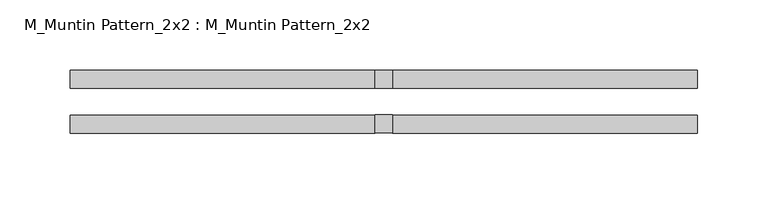
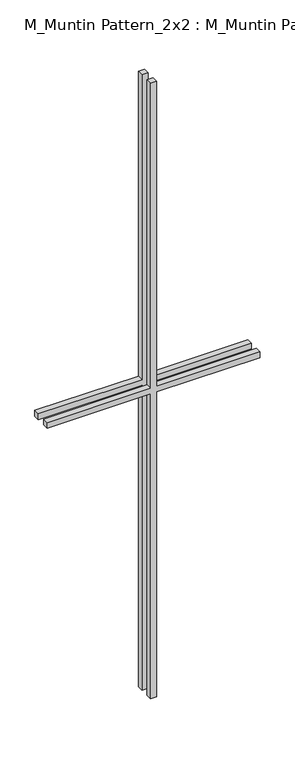
"""IFC4 building model written with IfcOpenShell, lengths in millimetres: proxy geometry, M_Muntin Pattern_2x2 : M_Muntin Pattern_2x2."""

from ifc_helpers import new_model, si_unit, frame, origin, place, context, project, spatial, polyline, outline, extrude, source, transform, mapped, element, save


def m_muntin_pattern_2x2_m_muntin_pattern_2x2_98e5798c(model_context):
    return source(origin(), model_context, "Body", "SweptSolid", [
        extrude(outline(polyline([(686.5, -6.35), (686.5, -223.0), (673.8, -223.0), (673.8, -6.35), (0.0, -6.35), (0.0, 6.35), (673.8, 6.35), (673.8, 223.0), (686.5, 223.0), (686.5, 6.35), (1360.3, 6.35), (1360.3, -6.35), (686.5, -6.35)])), frame((0.0, 9.525, 0.0), z_axis=(0.0, 1.0, 0.0), x_axis=(0.0, 0.0, 1.0)), (0.0, 0.0, 1.0), 12.7),
        extrude(outline(polyline([(686.5, -6.35), (686.5, -223.0), (673.8, -223.0), (673.8, -6.35), (0.0, -6.35), (0.0, 6.35), (673.8, 6.35), (673.8, 223.0), (686.5, 223.0), (686.5, 6.35), (1360.3, 6.35), (1360.3, -6.35), (686.5, -6.35)])), frame((0.0, -22.225, 0.0), z_axis=(0.0, 1.0, 0.0), x_axis=(0.0, 0.0, 1.0)), (0.0, 0.0, 1.0), 12.7),
    ])


if __name__ == "__main__":
    model = new_model("IFC4")
    model_context = context("Model", 3, world=origin())
    ifc_project = project(units=[si_unit("LENGTHUNIT", "METRE", prefix="MILLI")], contexts=[model_context])
    site = spatial("IfcSite", under=ifc_project)
    building = spatial("IfcBuilding", under=site)
    placement = place(None, origin())
    m_muntin_pattern_2x2_m_muntin_pattern_2x2_shape = m_muntin_pattern_2x2_m_muntin_pattern_2x2_98e5798c(model_context)
    element("IfcBuildingElementProxy", 1, Name="M_Muntin Pattern_2x2 : M_Muntin Pattern_2x2", ObjectType="M_Muntin Pattern_2x2 : M_Muntin Pattern_2x2", at=placement, inside=building, context=model_context, shape_type="MappedRepresentation", body=[
        mapped(m_muntin_pattern_2x2_m_muntin_pattern_2x2_shape, transform((0.0, 0.0, 0.0), x_axis=(1.0, 0.0, 0.0), y_axis=(0.0, 1.0, 0.0), z_axis=(0.0, 0.0, 1.0))),
    ])
    save(model, "model.ifc")

# Revit data of these elements
# Type "M_Muntin Pattern_2x2 : M_Muntin Pattern_2x2"
#   Width [instance default] = 1200 mm
#   Thickness = 12.7 mm
#   Height [instance default] = 1200 mm
#   Distance = 19.05 mm
#   Interior Material [instance default] = none
#   Exterior Material [instance default] = none
#   Default Elevation = 0
# Element 1 (IfcBuildingElementProxy, "M_Muntin Pattern_2x2 : M_Muntin Pattern_2x2")
#   Width = 446 mm
#   Height = 1360.3 mm
#   Interior Material = Wood - Stained
#   Exterior Material = Clad - White
#   Materials on its faces: "Clad - White", "Wood - Stained"
# Materials
#   "Clad - White": class "Wood", colour RGB 242 242 238, transparency 0, Cost = 0
#   "Wood - Stained": class "Wood", colour RGB 227 170 128, transparency 0, Cost = 0
